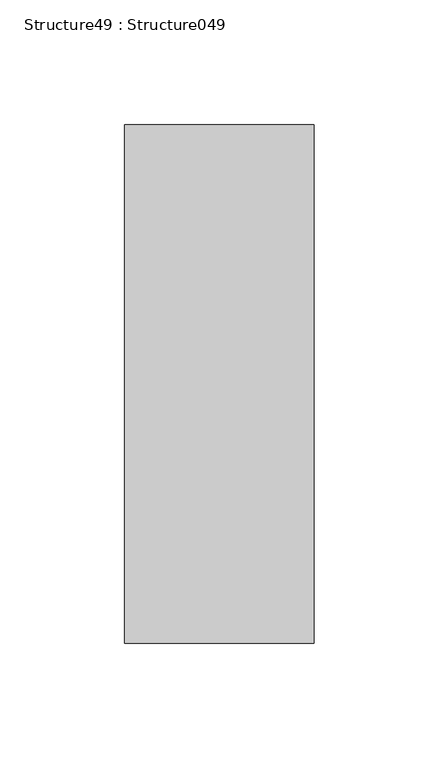
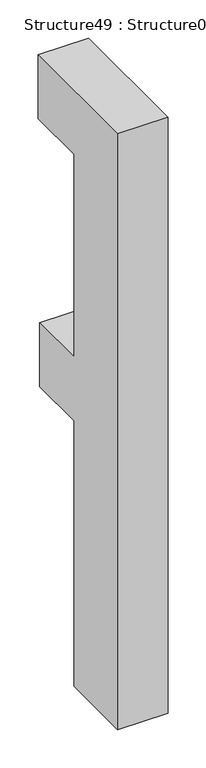
"""IFC4 building model written with IfcOpenShell, lengths in millimetres: proxy geometry, Structure49 : Structure049."""

from ifc_helpers import new_model, si_unit, frame, origin, place, context, project, spatial, polyline, outline, extrude, source, transform, mapped, element, save


def structure49_structure049_467c41e7(model_context):
    return source(origin(), model_context, "Body", "SweptSolid", [
        extrude(outline(polyline([(250386.3787026, 4480.4419946), (250594.4352235, 4480.4419946), (250594.4352235, 4378.4602217), (250500.614839, 4378.4602217), (250500.614839, 4054.8292705), (250590.3680696, 4054.8292705), (250590.3680696, 3952.8367913), (250500.614839, 3952.8367913), (250500.614839, 3528.5825142), (250386.3787026, 3528.5825142), (250386.3787026, 4480.4419946)])), frame((-38594.2176606, 0.0, 0.0), z_axis=(1.0, 0.0, 0.0), x_axis=(0.0, 1.0, 0.0)), (0.0, 0.0, 1.0), 76.2),
    ])


if __name__ == "__main__":
    model = new_model("IFC4")
    model_context = context("Model", 3, world=origin())
    ifc_project = project(units=[si_unit("LENGTHUNIT", "METRE", prefix="MILLI")], contexts=[model_context])
    site = spatial("IfcSite", under=ifc_project)
    building = spatial("IfcBuilding", under=site)
    placement = place(None, origin())
    structure49_structure049_shape = structure49_structure049_467c41e7(model_context)
    element("IfcBuildingElementProxy", 1, Name="Structure49 : Structure049", ObjectType="Structure49 : Structure049", at=placement, inside=building, context=model_context, shape_type="MappedRepresentation", body=[
        mapped(structure49_structure049_shape, transform((0.0, 0.0, 0.0), x_axis=(1.0, 0.0, 0.0), y_axis=(0.0, 1.0, 0.0), z_axis=(0.0, 0.0, 1.0))),
    ])
    save(model, "model.ifc")

# Revit data of these elements
# Type "Structure49 : Structure049"
#   NameOverride = "Structure049"
# Element 1 (IfcBuildingElementProxy, "Structure49 : Structure049")
#   Materials on its faces: "BRUSHED ALUM. LETTERING"
# Materials
#   "BRUSHED ALUM. LETTERING": class "Unassigned", colour RGB 169 181 186, transparency 0, Cost = 0
